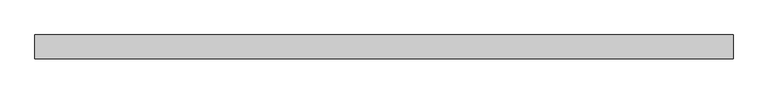
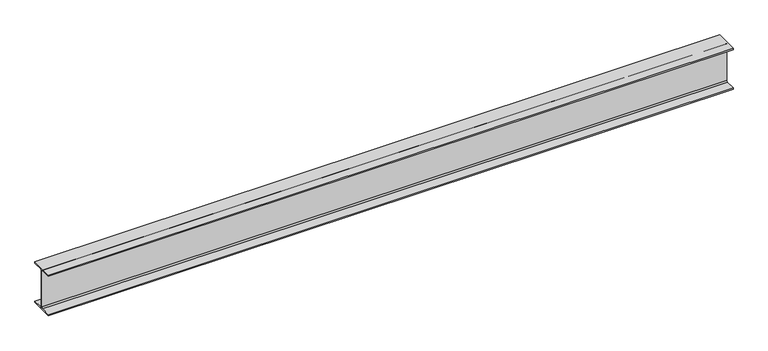
"""IFC4 building model written with IfcOpenShell, lengths in millimetres: beam geometry, Steel Beam_H-KSD3502 : H_SB_ASB_H-250x125x6x9."""

import ifcopenshell
import ifcopenshell.guid

model = None  # the IFC model being written
_history = None  # IfcOwnerHistory: only IFC2X3 demands one
_inside = {}  # id of a spatial element -> (the spatial element, [elements in it])
_under = {}  # id of a project, library or spatial element -> (it, [spatial elements below it])
_declared = {}  # id of a project -> (the project, [libraries it declares])
_typed = {}  # id of a type object -> (the type object, [elements of that type])
_made_of = {}  # id of a material, layer set ... -> (it, [elements and type objects made of it])


def new_model(schema):
    """Start an empty IFC model of exactly this schema.

    Asked for "IFC4X3", IfcOpenShell would pick the latest addendum, in which some entities
    have other attributes; the version numbers below select the first issue.
    IFC2X3 requires an IfcOwnerHistory on every rooted entity: one is made here for all.
    """
    global model, _history
    if schema == "IFC4X3":
        model = ifcopenshell.file(schema_version=(4, 3, 0, 0))
    else:
        model = ifcopenshell.file(schema=schema)
    _inside.clear()
    _under.clear()
    _declared.clear()
    _typed.clear()
    _made_of.clear()
    _history = None
    if model.schema == "IFC2X3":
        org = make("IfcOrganization", Name="unknown")
        user = make(
            "IfcPersonAndOrganization",
            ThePerson=make("IfcPerson", FamilyName="unknown"),
            TheOrganization=org,
        )
        app = make(
            "IfcApplication",
            ApplicationDeveloper=org,
            Version="unknown",
            ApplicationFullName="unknown",
            ApplicationIdentifier="unknown",
        )
        _history = make(
            "IfcOwnerHistory",
            OwningUser=user,
            OwningApplication=app,
            ChangeAction="ADDED",
            CreationDate=0,
        )
    return model


def make(cls, **values):
    """One entity of the class cls with the attributes given. An attribute that is None is left unset."""
    return model.create_entity(
        cls, **{name: value for name, value in values.items() if value is not None}
    )


def rooted(cls, **values):
    """An entity with a GlobalId (a new one), such as an element, a storey or a relation."""
    return make(cls, GlobalId=ifcopenshell.guid.new(), OwnerHistory=_history, **values)


def si_unit(unit_type, name, prefix=None):
    """IfcSIUnit, for example si_unit("LENGTHUNIT", "METRE", prefix="MILLI")."""
    return make("IfcSIUnit", UnitType=unit_type, Prefix=prefix, Name=name)


def assignment(units):
    """IfcUnitAssignment: the units of a project."""
    return None if units is None else make("IfcUnitAssignment", Units=units)


def point(xyz):
    """IfcCartesianPoint."""
    return None if xyz is None else make("IfcCartesianPoint", Coordinates=xyz)


def direction(xyz):
    """IfcDirection."""
    return None if xyz is None else make("IfcDirection", DirectionRatios=xyz)


def frame(location, z_axis=None, x_axis=None):
    """IfcAxis2Placement3D, a coordinate frame: its origin and axes. An axis left out is left unset."""
    return make(
        "IfcAxis2Placement3D",
        Location=point(location),
        Axis=direction(z_axis),
        RefDirection=direction(x_axis),
    )


def frame_2d(location, x_axis=None):
    """IfcAxis2Placement2D, a coordinate frame in the plane: its origin and x axis."""
    return make(
        "IfcAxis2Placement2D", Location=point(location), RefDirection=direction(x_axis)
    )


def origin():
    """The frame at (0, 0, 0) with its axes left unset."""
    return frame((0.0, 0.0, 0.0))


def place(relative_to, where):
    """IfcLocalPlacement: puts the frame where relative to a parent placement (None: the world)."""
    return make(
        "IfcLocalPlacement", PlacementRelTo=relative_to, RelativePlacement=where
    )


def context(
    kind, dimensions, precision=None, world=None, true_north=None, identifier=None
):
    """IfcGeometricRepresentationContext, for example the 3D "Model" context."""
    return make(
        "IfcGeometricRepresentationContext",
        ContextIdentifier=identifier,
        ContextType=kind,
        CoordinateSpaceDimension=dimensions,
        Precision=precision,
        WorldCoordinateSystem=world,
        TrueNorth=true_north,
    )


def project(units=None, contexts=None):
    """IfcProject with its units and contexts."""
    return rooted(
        "IfcProject",
        Name="project",
        RepresentationContexts=contexts,
        UnitsInContext=assignment(units),
    )


def spatial(cls, under=None, at=None, **own):
    """A site, building, storey or space (cls), placed at a placement, below another one or the project."""
    s = rooted(cls, ObjectPlacement=at, **own)
    if under is not None:
        _under.setdefault(under.id(), (under, []))[1].append(s)
    return s


def polyline(points):
    """IfcPolyline through the points."""
    return make("IfcPolyline", Points=[point(p) for p in points])


def circle_curve(where, radius):
    """IfcCircle in the frame where."""
    return make("IfcCircle", Position=where, Radius=radius)


def trimmed(basis, trim1, trim2, sense, master):
    """IfcTrimmedCurve: the piece of a basis curve between two trims."""
    return make(
        "IfcTrimmedCurve",
        BasisCurve=basis,
        Trim1=trim1,
        Trim2=trim2,
        SenseAgreement=sense,
        MasterRepresentation=master,
    )


def segment(curve, same_sense, transition):
    """IfcCompositeCurveSegment."""
    return make(
        "IfcCompositeCurveSegment",
        Transition=transition,
        SameSense=same_sense,
        ParentCurve=curve,
    )


def composite_curve(segments, self_intersect=None):
    """IfcCompositeCurve: segments joined end to end."""
    return make("IfcCompositeCurve", Segments=segments, SelfIntersect=self_intersect)


def outline(outer, holes=None, kind="AREA"):
    """IfcArbitraryClosedProfileDef: a profile drawn as a closed curve; with holes, ...WithVoids."""
    if holes is None:
        return make("IfcArbitraryClosedProfileDef", ProfileType=kind, OuterCurve=outer)
    return make(
        "IfcArbitraryProfileDefWithVoids",
        ProfileType=kind,
        OuterCurve=outer,
        InnerCurves=holes,
    )


def extrude(swept, where, along, depth):
    """IfcExtrudedAreaSolid: the profile swept, set in the frame where, extruded along a direction by depth."""
    return make(
        "IfcExtrudedAreaSolid",
        SweptArea=swept,
        Position=where,
        ExtrudedDirection=direction(along),
        Depth=depth,
    )


def shape(context_of_items, identifier, shape_type, items):
    """IfcShapeRepresentation: the items that make up one representation, for example the "Body"."""
    return make(
        "IfcShapeRepresentation",
        ContextOfItems=context_of_items,
        RepresentationIdentifier=identifier,
        RepresentationType=shape_type,
        Items=items,
    )


def source(mapping_origin, context_of_items, identifier, shape_type, items):
    """IfcRepresentationMap: a shape defined once, which mapped items show again and again."""
    return make(
        "IfcRepresentationMap",
        MappingOrigin=mapping_origin,
        MappedRepresentation=shape(context_of_items, identifier, shape_type, items),
    )


def transform(
    local_origin,
    x_axis=None,
    y_axis=None,
    z_axis=None,
    scale=None,
    scale2=None,
    scale3=None,
    uniform=True,
):
    """IfcCartesianTransformationOperator3D, or its non-uniform kind. x_axis, y_axis, z_axis: its Axis1, 2, 3."""
    if uniform:
        return make(
            "IfcCartesianTransformationOperator3D",
            Axis1=direction(x_axis),
            Axis2=direction(y_axis),
            LocalOrigin=point(local_origin),
            Scale=scale,
            Axis3=direction(z_axis),
        )
    return make(
        "IfcCartesianTransformationOperator3DnonUniform",
        Axis1=direction(x_axis),
        Axis2=direction(y_axis),
        LocalOrigin=point(local_origin),
        Scale=scale,
        Axis3=direction(z_axis),
        Scale2=scale2,
        Scale3=scale3,
    )


def mapped(mapping_source, mapping_target):
    """IfcMappedItem: shows the shape of a source again, moved by a transform."""
    return make(
        "IfcMappedItem", MappingSource=mapping_source, MappingTarget=mapping_target
    )


def made_of(thing, what):
    """Note that an element or type object is made of a material, layer set ...; save() writes the relation."""
    if what is not None:
        _made_of.setdefault(what.id(), (what, []))[1].append(thing)
    return thing


def element(
    cls,
    number,
    at=None,
    inside=None,
    cuts=None,
    type_object=None,
    material=None,
    context=None,
    identifier="Body",
    shape_type=None,
    held_by="IfcProductDefinitionShape",
    body=None,
    shapes=None,
    **own,
):
    """One element of the class cls, such as IfcWall. Its Tag is "e" and its number.

    at: its placement. inside: the storey or other place that contains it. cuts: it is an
    opening in that element (IfcRelVoidsElement). A single representation is given by context,
    identifier, shape_type and body (its items); several are given by shapes. held_by: the class
    of the entity that holds the representations. save() writes the other relations.
    """
    e = rooted(cls, Tag="e%d" % number, ObjectPlacement=at, **own)
    if body is not None:
        shapes = [shape(context, identifier, shape_type, body)]
    if shapes is not None:
        e.Representation = make(held_by, Representations=shapes)
    if inside is not None:
        _inside.setdefault(inside.id(), (inside, []))[1].append(e)
    if cuts is not None:
        rooted(
            "IfcRelVoidsElement", RelatingBuildingElement=cuts, RelatedOpeningElement=e
        )
    if type_object is not None:
        _typed.setdefault(type_object.id(), (type_object, []))[1].append(e)
    return made_of(e, material)


def aggregate(whole, parts):
    """IfcRelAggregates: a whole, such as a stair, and the parts it consists of."""
    return rooted("IfcRelAggregates", RelatingObject=whole, RelatedObjects=parts)


def save(model, path):
    """Write the relations noted so far, then the file.

    IfcRelAggregates (storeys below a building ...), IfcRelContainedInSpatialStructure (elements
    in a storey), IfcRelDefinesByType, IfcRelAssociatesMaterial and IfcRelDeclares: one each for
    every whole, place, type object, material and project.
    """
    for whole, parts in _under.values():
        aggregate(whole, parts)
    for where, things in _inside.values():
        rooted(
            "IfcRelContainedInSpatialStructure",
            RelatedElements=things,
            RelatingStructure=where,
        )
    for kind, things in _typed.values():
        rooted("IfcRelDefinesByType", RelatedObjects=things, RelatingType=kind)
    for what, things in _made_of.values():
        rooted("IfcRelAssociatesMaterial", RelatedObjects=things, RelatingMaterial=what)
    for by, libraries in _declared.values():
        rooted("IfcRelDeclares", RelatingContext=by, RelatedDefinitions=libraries)
    model.write(path)


def beam_54c8535d(model_context):
    return source(origin(), model_context, "Body", "SweptSolid", [
        extrude(outline(composite_curve([segment(polyline([(82.5, -141.5), (82.5, -151.7), (-82.5, -151.7), (-82.5, -141.5), (-11.9, -141.5)]), True, "CONTINUOUS"), segment(trimmed(circle_curve(frame_2d((-11.9, -132.6)), 8.9), [point((-11.9, -141.5))], [point((-3.0, -132.6))], True, "CARTESIAN"), True, "CONTINUOUS"), segment(polyline([(-3.0, -132.6), (-3.0, 132.6)]), True, "CONTINUOUS"), segment(trimmed(circle_curve(frame_2d((-11.9, 132.6)), 8.9), [point((-3.0, 132.6))], [point((-11.9, 141.5))], True, "CARTESIAN"), True, "CONTINUOUS"), segment(polyline([(-11.9, 141.5), (-82.5, 141.5), (-82.5, 151.7), (82.5, 151.7), (82.5, 141.5), (11.9, 141.5)]), True, "CONTINUOUS"), segment(trimmed(circle_curve(frame_2d((11.9, 132.6)), 8.9), [point((11.9, 141.5))], [point((3.0, 132.6))], True, "CARTESIAN"), True, "CONTINUOUS"), segment(polyline([(3.0, 132.6), (3.0, -132.6)]), True, "CONTINUOUS"), segment(trimmed(circle_curve(frame_2d((11.9, -132.6)), 8.9), [point((3.0, -132.6))], [point((11.9, -141.5))], True, "CARTESIAN"), True, "CONTINUOUS"), segment(polyline([(11.9, -141.5), (82.5, -141.5)]), True, "CONTINUOUS")], self_intersect=False)), frame((-2403.3634808, 0.0, 0.0), z_axis=(1.0, 0.0, 0.0), x_axis=(0.0, 1.0, 0.0)), (0.0, 0.0, 1.0), 4815.6934866),
    ])


if __name__ == "__main__":
    model = new_model("IFC4")
    model_context = context("Model", 3, world=origin())
    ifc_project = project(units=[si_unit("LENGTHUNIT", "METRE", prefix="MILLI")], contexts=[model_context])
    site = spatial("IfcSite", under=ifc_project)
    building = spatial("IfcBuilding", under=site)
    placement = place(None, origin())
    beam_shape = beam_54c8535d(model_context)
    element("IfcBeam", 1, ObjectType="Steel Beam_H-KSD3502 : H_SB_ASB_H-250x125x6x9", at=placement, inside=building, context=model_context, shape_type="MappedRepresentation", body=[
        mapped(beam_shape, transform((0.0, 0.0, 0.0), x_axis=(1.0, 0.0, 0.0), y_axis=(0.0, 1.0, 0.0), z_axis=(0.0, 0.0, 1.0))),
    ])
    save(model, "model.ifc")

# Revit data of these elements
# Type "Steel Beam_H-KSD3502 : H_SB_ASB_H-250x125x6x9"
#   Width = 12.5 cm
#   Web Thickness = 0.6 cm
#   Web Fillet = 1.2 cm
#   Warping Constant = 42539.8 cm⁶
#   Torsional Moment of Inertia = 7.8102 cm⁴
#   Torsional Modulus = 1.0 cm³
#   Section Area = 37.66 cm²
#   Plastic Modulus weak axis = 73.1 cm³
#   Plastic Modulus strong axis = 366.0 cm³
#   Perimeter = 0.97 m²/m
#   Nominal Weight = 29.60 kgf/m
#   Moment of Inertia weak axis = 294.00 cm⁴
#   Moment of Inertia strong axis = 4050.00 cm⁴
#   Height = 25.0 cm
#   Flange Thickness = 0.9 cm
#   Elastic Modulus weak axis = 47.0 cm³
#   Elastic Modulus strong axis = 324.0 cm³
#   Centroid Vertical = 12.5 cm
#   Centroid Horizontal = 6.25 cm
#   Length [instance default] = 1.5240 m
#   Structural Material [instance default] = Steel, 45-345
#   Assembly Code = ""
# Element 1 (IfcBeam, "Steel Beam_H-KSD3502 : H_SB_ASB_H-250x125x6x9")
#   Structural Material = none
# Materials
#   "Steel, 45-345": class "Metal", colour RGB 189 187 185, transparency 0, Description = "Steel 345 MPa", Cost = 0
